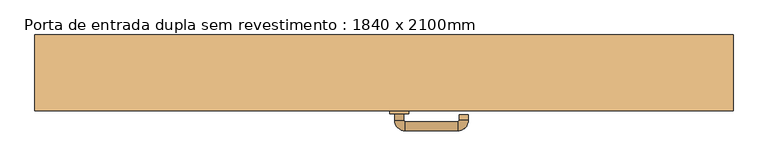
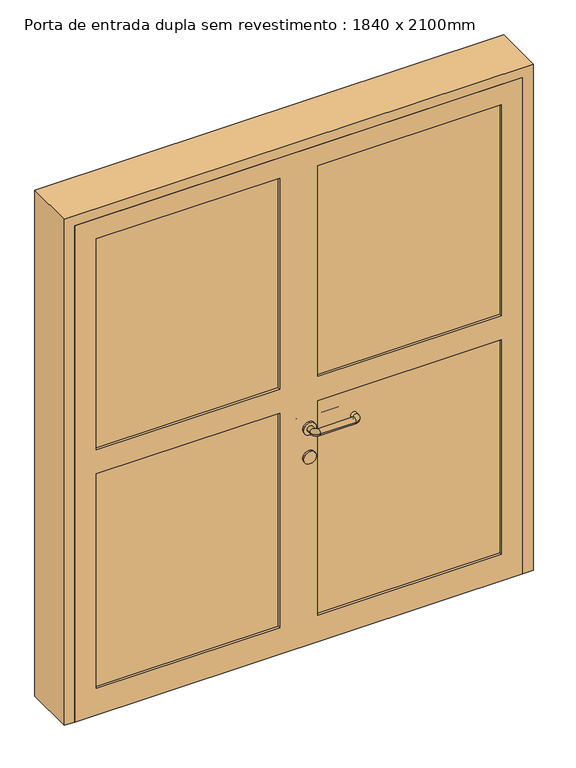
"""IFC4 building model written with IfcOpenShell, lengths in millimetres: door geometry, Porta de entrada dupla sem revestimento : 1840 x 2100mm."""

import ifcopenshell
import ifcopenshell.guid

model = None  # the IFC model being written
_history = None  # IfcOwnerHistory: only IFC2X3 demands one
_inside = {}  # id of a spatial element -> (the spatial element, [elements in it])
_under = {}  # id of a project, library or spatial element -> (it, [spatial elements below it])
_declared = {}  # id of a project -> (the project, [libraries it declares])
_typed = {}  # id of a type object -> (the type object, [elements of that type])
_made_of = {}  # id of a material, layer set ... -> (it, [elements and type objects made of it])


def new_model(schema):
    """Start an empty IFC model of exactly this schema.

    Asked for "IFC4X3", IfcOpenShell would pick the latest addendum, in which some entities
    have other attributes; the version numbers below select the first issue.
    IFC2X3 requires an IfcOwnerHistory on every rooted entity: one is made here for all.
    """
    global model, _history
    if schema == "IFC4X3":
        model = ifcopenshell.file(schema_version=(4, 3, 0, 0))
    else:
        model = ifcopenshell.file(schema=schema)
    _inside.clear()
    _under.clear()
    _declared.clear()
    _typed.clear()
    _made_of.clear()
    _history = None
    if model.schema == "IFC2X3":
        org = make("IfcOrganization", Name="unknown")
        user = make(
            "IfcPersonAndOrganization",
            ThePerson=make("IfcPerson", FamilyName="unknown"),
            TheOrganization=org,
        )
        app = make(
            "IfcApplication",
            ApplicationDeveloper=org,
            Version="unknown",
            ApplicationFullName="unknown",
            ApplicationIdentifier="unknown",
        )
        _history = make(
            "IfcOwnerHistory",
            OwningUser=user,
            OwningApplication=app,
            ChangeAction="ADDED",
            CreationDate=0,
        )
    return model


def make(cls, **values):
    """One entity of the class cls with the attributes given. An attribute that is None is left unset."""
    return model.create_entity(
        cls, **{name: value for name, value in values.items() if value is not None}
    )


def rooted(cls, **values):
    """An entity with a GlobalId (a new one), such as an element, a storey or a relation."""
    return make(cls, GlobalId=ifcopenshell.guid.new(), OwnerHistory=_history, **values)


def si_unit(unit_type, name, prefix=None):
    """IfcSIUnit, for example si_unit("LENGTHUNIT", "METRE", prefix="MILLI")."""
    return make("IfcSIUnit", UnitType=unit_type, Prefix=prefix, Name=name)


def assignment(units):
    """IfcUnitAssignment: the units of a project."""
    return None if units is None else make("IfcUnitAssignment", Units=units)


def point(xyz):
    """IfcCartesianPoint."""
    return None if xyz is None else make("IfcCartesianPoint", Coordinates=xyz)


def direction(xyz):
    """IfcDirection."""
    return None if xyz is None else make("IfcDirection", DirectionRatios=xyz)


def frame(location, z_axis=None, x_axis=None):
    """IfcAxis2Placement3D, a coordinate frame: its origin and axes. An axis left out is left unset."""
    return make(
        "IfcAxis2Placement3D",
        Location=point(location),
        Axis=direction(z_axis),
        RefDirection=direction(x_axis),
    )


def frame_2d(location, x_axis=None):
    """IfcAxis2Placement2D, a coordinate frame in the plane: its origin and x axis."""
    return make(
        "IfcAxis2Placement2D", Location=point(location), RefDirection=direction(x_axis)
    )


def origin():
    """The frame at (0, 0, 0) with its axes left unset."""
    return frame((0.0, 0.0, 0.0))


def place(relative_to, where):
    """IfcLocalPlacement: puts the frame where relative to a parent placement (None: the world)."""
    return make(
        "IfcLocalPlacement", PlacementRelTo=relative_to, RelativePlacement=where
    )


def context(
    kind, dimensions, precision=None, world=None, true_north=None, identifier=None
):
    """IfcGeometricRepresentationContext, for example the 3D "Model" context."""
    return make(
        "IfcGeometricRepresentationContext",
        ContextIdentifier=identifier,
        ContextType=kind,
        CoordinateSpaceDimension=dimensions,
        Precision=precision,
        WorldCoordinateSystem=world,
        TrueNorth=true_north,
    )


def project(units=None, contexts=None):
    """IfcProject with its units and contexts."""
    return rooted(
        "IfcProject",
        Name="project",
        RepresentationContexts=contexts,
        UnitsInContext=assignment(units),
    )


def spatial(cls, under=None, at=None, **own):
    """A site, building, storey or space (cls), placed at a placement, below another one or the project."""
    s = rooted(cls, ObjectPlacement=at, **own)
    if under is not None:
        _under.setdefault(under.id(), (under, []))[1].append(s)
    return s


def polyline(points):
    """IfcPolyline through the points."""
    return make("IfcPolyline", Points=[point(p) for p in points])


def circle_curve(where, radius):
    """IfcCircle in the frame where."""
    return make("IfcCircle", Position=where, Radius=radius)


def ellipse_curve(where, semi_axis1, semi_axis2):
    """IfcEllipse in the frame where."""
    return make(
        "IfcEllipse", Position=where, SemiAxis1=semi_axis1, SemiAxis2=semi_axis2
    )


def trimmed(basis, trim1, trim2, sense, master):
    """IfcTrimmedCurve: the piece of a basis curve between two trims."""
    return make(
        "IfcTrimmedCurve",
        BasisCurve=basis,
        Trim1=trim1,
        Trim2=trim2,
        SenseAgreement=sense,
        MasterRepresentation=master,
    )


def segment(curve, same_sense, transition):
    """IfcCompositeCurveSegment."""
    return make(
        "IfcCompositeCurveSegment",
        Transition=transition,
        SameSense=same_sense,
        ParentCurve=curve,
    )


def composite_curve(segments, self_intersect=None):
    """IfcCompositeCurve: segments joined end to end."""
    return make("IfcCompositeCurve", Segments=segments, SelfIntersect=self_intersect)


def outline(outer, holes=None, kind="AREA"):
    """IfcArbitraryClosedProfileDef: a profile drawn as a closed curve; with holes, ...WithVoids."""
    if holes is None:
        return make("IfcArbitraryClosedProfileDef", ProfileType=kind, OuterCurve=outer)
    return make(
        "IfcArbitraryProfileDefWithVoids",
        ProfileType=kind,
        OuterCurve=outer,
        InnerCurves=holes,
    )


def extrude(swept, where, along, depth):
    """IfcExtrudedAreaSolid: the profile swept, set in the frame where, extruded along a direction by depth."""
    return make(
        "IfcExtrudedAreaSolid",
        SweptArea=swept,
        Position=where,
        ExtrudedDirection=direction(along),
        Depth=depth,
    )


def faces_of(points, faces, orient=None, outer=None):
    """IfcFace entities. A face is a list of loops; a loop is a list of indices into points, from 0.

    orient and outer hold one flag for each loop. By default every Orientation is true, the
    first loop of a face is its IfcFaceOuterBound and the others are IfcFaceBound.
    """
    made = []
    for i, loops in enumerate(faces):
        bounds = []
        for j, loop in enumerate(loops):
            is_outer = j == 0 if outer is None else outer[i][j]
            bounds.append(
                make(
                    "IfcFaceOuterBound" if is_outer else "IfcFaceBound",
                    Bound=make("IfcPolyLoop", Polygon=[points[k] for k in loop]),
                    Orientation=True if orient is None else orient[i][j],
                )
            )
        made.append(make("IfcFace", Bounds=bounds))
    return made


def faceted_brep(points, faces, orient=None, outer=None, voids=None):
    """IfcFacetedBrep: a solid bounded by flat faces; with voids (closed shells), ...WithVoids."""
    shared = [point(p) for p in points]
    hull = make("IfcClosedShell", CfsFaces=faces_of(shared, faces, orient, outer))
    if voids is None:
        return make("IfcFacetedBrep", Outer=hull)
    return make(
        "IfcFacetedBrepWithVoids",
        Outer=hull,
        Voids=[
            make(cls, CfsFaces=faces_of(shared, fs, o, b)) for cls, fs, o, b in voids
        ],
    )


def shape(context_of_items, identifier, shape_type, items):
    """IfcShapeRepresentation: the items that make up one representation, for example the "Body"."""
    return make(
        "IfcShapeRepresentation",
        ContextOfItems=context_of_items,
        RepresentationIdentifier=identifier,
        RepresentationType=shape_type,
        Items=items,
    )


def source(mapping_origin, context_of_items, identifier, shape_type, items):
    """IfcRepresentationMap: a shape defined once, which mapped items show again and again."""
    return make(
        "IfcRepresentationMap",
        MappingOrigin=mapping_origin,
        MappedRepresentation=shape(context_of_items, identifier, shape_type, items),
    )


def transform(
    local_origin,
    x_axis=None,
    y_axis=None,
    z_axis=None,
    scale=None,
    scale2=None,
    scale3=None,
    uniform=True,
):
    """IfcCartesianTransformationOperator3D, or its non-uniform kind. x_axis, y_axis, z_axis: its Axis1, 2, 3."""
    if uniform:
        return make(
            "IfcCartesianTransformationOperator3D",
            Axis1=direction(x_axis),
            Axis2=direction(y_axis),
            LocalOrigin=point(local_origin),
            Scale=scale,
            Axis3=direction(z_axis),
        )
    return make(
        "IfcCartesianTransformationOperator3DnonUniform",
        Axis1=direction(x_axis),
        Axis2=direction(y_axis),
        LocalOrigin=point(local_origin),
        Scale=scale,
        Axis3=direction(z_axis),
        Scale2=scale2,
        Scale3=scale3,
    )


def mapped(mapping_source, mapping_target):
    """IfcMappedItem: shows the shape of a source again, moved by a transform."""
    return make(
        "IfcMappedItem", MappingSource=mapping_source, MappingTarget=mapping_target
    )


def made_of(thing, what):
    """Note that an element or type object is made of a material, layer set ...; save() writes the relation."""
    if what is not None:
        _made_of.setdefault(what.id(), (what, []))[1].append(thing)
    return thing


def element(
    cls,
    number,
    at=None,
    inside=None,
    cuts=None,
    type_object=None,
    material=None,
    context=None,
    identifier="Body",
    shape_type=None,
    held_by="IfcProductDefinitionShape",
    body=None,
    shapes=None,
    **own,
):
    """One element of the class cls, such as IfcWall. Its Tag is "e" and its number.

    at: its placement. inside: the storey or other place that contains it. cuts: it is an
    opening in that element (IfcRelVoidsElement). A single representation is given by context,
    identifier, shape_type and body (its items); several are given by shapes. held_by: the class
    of the entity that holds the representations. save() writes the other relations.
    """
    e = rooted(cls, Tag="e%d" % number, ObjectPlacement=at, **own)
    if body is not None:
        shapes = [shape(context, identifier, shape_type, body)]
    if shapes is not None:
        e.Representation = make(held_by, Representations=shapes)
    if inside is not None:
        _inside.setdefault(inside.id(), (inside, []))[1].append(e)
    if cuts is not None:
        rooted(
            "IfcRelVoidsElement", RelatingBuildingElement=cuts, RelatedOpeningElement=e
        )
    if type_object is not None:
        _typed.setdefault(type_object.id(), (type_object, []))[1].append(e)
    return made_of(e, material)


def aggregate(whole, parts):
    """IfcRelAggregates: a whole, such as a stair, and the parts it consists of."""
    return rooted("IfcRelAggregates", RelatingObject=whole, RelatedObjects=parts)


def save(model, path):
    """Write the relations noted so far, then the file.

    IfcRelAggregates (storeys below a building ...), IfcRelContainedInSpatialStructure (elements
    in a storey), IfcRelDefinesByType, IfcRelAssociatesMaterial and IfcRelDeclares: one each for
    every whole, place, type object, material and project.
    """
    for whole, parts in _under.values():
        aggregate(whole, parts)
    for where, things in _inside.values():
        rooted(
            "IfcRelContainedInSpatialStructure",
            RelatedElements=things,
            RelatingStructure=where,
        )
    for kind, things in _typed.values():
        rooted("IfcRelDefinesByType", RelatedObjects=things, RelatingType=kind)
    for what, things in _made_of.values():
        rooted("IfcRelAssociatesMaterial", RelatedObjects=things, RelatingMaterial=what)
    for by, libraries in _declared.values():
        rooted("IfcRelDeclares", RelatingContext=by, RelatedDefinitions=libraries)
    model.write(path)


def plane_surface(at):
    """IfcPlane: the flat surface through the origin of the frame at, square to its z axis."""
    return make("IfcPlane", Position=at)


def cylinder_surface(at, radius):
    """IfcCylindricalSurface: all points at the distance radius from the z axis of the frame at."""
    return make("IfcCylindricalSurface", Position=at, Radius=radius)


def revolved_surface(curve, axis_point, axis_direction):
    """IfcSurfaceOfRevolution: the curve turned about the line through axis_point along axis_direction."""
    return make(
        "IfcSurfaceOfRevolution",
        SweptCurve=make("IfcArbitraryOpenProfileDef", ProfileType="CURVE", Curve=curve),
        AxisPosition=make("IfcAxis1Placement", Location=point(axis_point), Axis=direction(axis_direction)),
    )


def advanced_brep(points, edges, surfaces, faces):
    """IfcAdvancedBrep: a solid bounded by faces that lie on surfaces and meet in shared edges.

    An edge is (start, end): straight between two places in points (the first is 0);
    or (start, end, curve); or (start, end, curve, False) where it runs against its curve.
    A face is (place in surfaces, loops), or (place, loops, False) where it looks against
    its surface's normal. A loop lists edges by number (the first is 1), with a minus sign
    where the edge is run from its end to its start. The first loop is the outer one.
    """
    corners = [point(p) for p in points]
    vertices = [make("IfcVertexPoint", VertexGeometry=c) for c in corners]
    made = []
    for start, end, *more in edges:
        made.append(
            make(
                "IfcEdgeCurve",
                EdgeStart=vertices[start],
                EdgeEnd=vertices[end],
                EdgeGeometry=more[0] if more else make("IfcPolyline", Points=[corners[start], corners[end]]),
                SameSense=more[1] if len(more) > 1 else True,
            )
        )
    hull = []
    for where, loops, *sense in faces:
        bounds = []
        for j, loop in enumerate(loops):
            ring = [make("IfcOrientedEdge", EdgeElement=made[abs(k) - 1], Orientation=k > 0) for k in loop]
            bounds.append(
                make(
                    "IfcFaceOuterBound" if j == 0 else "IfcFaceBound",
                    Bound=make("IfcEdgeLoop", EdgeList=ring),
                    Orientation=True,
                )
            )
        hull.append(make("IfcAdvancedFace", Bounds=bounds, FaceSurface=surfaces[where], SameSense=sense[0] if sense else True))
    return make("IfcAdvancedBrep", Outer=make("IfcClosedShell", CfsFaces=hull))


def porta_de_entrada_dupla_sem_revestimento_1840_x_2100mm_60e580c7(model_context):
    return source(origin(), model_context, "Body", "SolidModel", [
        advanced_brep(
        [(52.0, -57.0, 900.0), (28.0, -57.0, 900.0), (52.0, -40.0, 900.0), (28.0, -40.0, 900.0), (55.0, -13.0, 900.0), (55.0, -37.0, 900.0), (195.0, -37.0, 900.0), (195.0, -13.0, 900.0), (222.0, -40.0, 900.0), (198.0, -40.0, 900.0), (198.0, -55.0, 900.0), (222.0, -55.0, 900.0)],
        [
            (0, 1, circle_curve(frame((40.0, -57.0, 900.0), z_axis=(0.0, -1.0, 0.0), x_axis=(-1.0, 0.0, 0.0)), 12.0)),
            (1, 0, circle_curve(frame((40.0, -57.0, 900.0), z_axis=(0.0, -1.0, 0.0), x_axis=(-1.0, 0.0, 0.0)), 12.0)),
            (0, 2),
            (2, 3, circle_curve(frame((40.0, -40.0, 900.0), z_axis=(0.0, -1.0, 0.0), x_axis=(-1.0, 0.0, 0.0)), 12.0)),
            (3, 1),
            (3, 2, circle_curve(frame((40.0, -40.0, 900.0), z_axis=(0.0, -1.0, 0.0), x_axis=(-1.0, 0.0, 0.0)), 12.0)),
            (4, 3, circle_curve(frame((55.0, -40.0, 900.0), z_axis=(0.0, 0.0, 1.0), x_axis=(-1.0, 0.0, 0.0)), 27.0)),
            (2, 5, circle_curve(frame((55.0, -40.0, 900.0), z_axis=(0.0, 0.0, -1.0), x_axis=(-1.0, 0.0, 0.0)), 3.0)),
            (5, 4, circle_curve(frame((55.0, -25.0, 900.0), z_axis=(-1.0, 0.0, 0.0), x_axis=(0.0, 1.0, 0.0)), 12.0)),
            (4, 5, circle_curve(frame((55.0, -25.0, 900.0), z_axis=(-1.0, 0.0, 0.0), x_axis=(0.0, 1.0, 0.0)), 12.0)),
            (5, 6),
            (6, 7, circle_curve(frame((195.0, -25.0, 900.0), z_axis=(-1.0, 0.0, 0.0), x_axis=(0.0, 1.0, 0.0)), 12.0)),
            (7, 4),
            (7, 6, circle_curve(frame((195.0, -25.0, 900.0), z_axis=(-1.0, 0.0, 0.0), x_axis=(0.0, 1.0, 0.0)), 12.0)),
            (8, 7, circle_curve(frame((195.0, -40.0, 900.0), z_axis=(0.0, 0.0, 1.0), x_axis=(0.0, 1.0, 0.0)), 27.0)),
            (6, 9, circle_curve(frame((195.0, -40.0, 900.0), z_axis=(0.0, 0.0, -1.0), x_axis=(0.0, 1.0, 0.0)), 3.0)),
            (9, 8, circle_curve(frame((210.0, -40.0, 900.0), z_axis=(0.0, 1.0, 0.0), x_axis=(1.0, 0.0, 0.0)), 12.0)),
            (8, 9, circle_curve(frame((210.0, -40.0, 900.0), z_axis=(0.0, 1.0, 0.0), x_axis=(1.0, 0.0, 0.0)), 12.0)),
            (10, 11, circle_curve(frame((210.0, -55.0, 900.0), z_axis=(0.0, -1.0, 0.0), x_axis=(1.0, 0.0, 0.0)), 12.0)),
            (11, 10, circle_curve(frame((210.0, -55.0, 900.0), z_axis=(0.0, -1.0, 0.0), x_axis=(1.0, 0.0, 0.0)), 12.0)),
            (9, 10),
            (11, 8),
        ],
        [
            plane_surface(frame((-802.0, -57.0, 1730.0), z_axis=(0.0, -1.0, 0.0), x_axis=(0.0, 0.0, 1.0))),
            cylinder_surface(frame((40.0, -57.0, 900.0), z_axis=(0.0, -1.0, 0.0), x_axis=(-1.0, 0.0, 0.0)), 12.0),
            revolved_surface(trimmed(ellipse_curve(frame((40.0, -40.0, 900.0), z_axis=(0.0, -1.0, 0.0), x_axis=(-1.0, 0.0, 0.0)), 12.0, 12.0), [point((52.0, -40.0, 900.0))], [point((28.0, -40.0, 900.0))], True, "CARTESIAN"), (55.0, -40.0, 1730.0), (0.0, 0.0, -1.0)),
            revolved_surface(trimmed(ellipse_curve(frame((40.0, -40.0, 900.0), z_axis=(0.0, -1.0, 0.0), x_axis=(-1.0, 0.0, 0.0)), 12.0, 12.0), [point((28.0, -40.0, 900.0))], [point((52.0, -40.0, 900.0))], True, "CARTESIAN"), (55.0, -40.0, 1730.0), (0.0, 0.0, -1.0)),
            cylinder_surface(frame((55.0, -25.0, 900.0), z_axis=(-1.0, 0.0, 0.0), x_axis=(0.0, 1.0, 0.0)), 12.0),
            revolved_surface(trimmed(ellipse_curve(frame((195.0, -25.0, 900.0), z_axis=(-1.0, 0.0, 0.0), x_axis=(0.0, 1.0, 0.0)), 12.0, 12.0), [point((195.0, -37.0, 900.0))], [point((195.0, -13.0, 900.0))], True, "CARTESIAN"), (195.0, -40.0, 1730.0), (0.0, 0.0, -1.0)),
            revolved_surface(trimmed(ellipse_curve(frame((195.0, -25.0, 900.0), z_axis=(-1.0, 0.0, 0.0), x_axis=(0.0, 1.0, 0.0)), 12.0, 12.0), [point((195.0, -13.0, 900.0))], [point((195.0, -37.0, 900.0))], True, "CARTESIAN"), (195.0, -40.0, 1730.0), (0.0, 0.0, -1.0)),
            plane_surface(frame((-632.0, -55.0, 1730.0), z_axis=(0.0, -1.0, 0.0), x_axis=(0.0, 0.0, -1.0))),
            cylinder_surface(frame((210.0, -40.0, 900.0), z_axis=(0.0, 1.0, 0.0), x_axis=(1.0, 0.0, 0.0)), 12.0),
        ],
        [
            (0, [[1, 2]]),
            (1, [[-1, 3, 4, 5]]),
            (1, [[-2, -5, 6, -3]]),
            (2, [[7, -4, 8, 9]]),
            (3, [[-8, -6, -7, 10]]),
            (4, [[-9, 11, 12, 13]]),
            (4, [[-10, -13, 14, -11]]),
            (5, [[15, -12, 16, 17]]),
            (6, [[-16, -14, -15, 18]]),
            (7, [[19, 20]]),
            (8, [[-17, 21, -20, 22]]),
            (8, [[-18, -22, -19, -21]]),
        ],
    ),
        extrude(outline(composite_curve([segment(trimmed(circle_curve(frame_2d((780.0, 40.0)), 25.0), [point((780.0, 15.0))], [point((780.0, 65.0))], False, "CARTESIAN"), True, "CONTINUOUS"), segment(trimmed(circle_curve(frame_2d((780.0, 40.0)), 25.0), [point((780.0, 65.0))], [point((780.0, 15.0))], False, "CARTESIAN"), True, "CONTINUOUS")], self_intersect=False)), frame((0.0, -65.0, 0.0), z_axis=(0.0, 1.0, 0.0), x_axis=(0.0, 0.0, 1.0)), (0.0, 0.0, 1.0), 8.0),
        extrude(outline(composite_curve([segment(trimmed(circle_curve(frame_2d((900.0, 40.0)), 25.0), [point((900.0, 15.0))], [point((900.0, 65.0))], False, "CARTESIAN"), True, "CONTINUOUS"), segment(trimmed(circle_curve(frame_2d((900.0, 40.0)), 25.0), [point((900.0, 65.0))], [point((900.0, 15.0))], False, "CARTESIAN"), True, "CONTINUOUS")], self_intersect=False)), frame((0.0, -65.0, 0.0), z_axis=(0.0, 1.0, 0.0), x_axis=(0.0, 0.0, 1.0)), (0.0, 0.0, 1.0), 8.0),
        advanced_brep(
        [(28.0, -108.0, 900.0), (52.0, -108.0, 900.0), (28.0, -125.0, 900.0), (52.0, -125.0, 900.0), (55.0, -128.0, 900.0), (55.0, -152.0, 900.0), (195.0, -152.0, 900.0), (195.0, -128.0, 900.0), (198.0, -125.0, 900.0), (222.0, -125.0, 900.0), (222.0, -110.0, 900.0), (198.0, -110.0, 900.0)],
        [
            (0, 1, circle_curve(frame((40.0, -108.0, 900.0), z_axis=(0.0, 1.0, 0.0), x_axis=(1.0, 0.0, 0.0)), 12.0)),
            (1, 0, circle_curve(frame((40.0, -108.0, 900.0), z_axis=(0.0, 1.0, 0.0), x_axis=(1.0, 0.0, 0.0)), 12.0)),
            (0, 2),
            (2, 3, circle_curve(frame((40.0, -125.0, 900.0), z_axis=(0.0, 1.0, 0.0), x_axis=(1.0, 0.0, 0.0)), 12.0)),
            (3, 1),
            (3, 2, circle_curve(frame((40.0, -125.0, 900.0), z_axis=(0.0, 1.0, 0.0), x_axis=(1.0, 0.0, 0.0)), 12.0)),
            (4, 3, circle_curve(frame((55.0, -125.0, 900.0), z_axis=(0.0, 0.0, -1.0), x_axis=(-1.0, 0.0, 0.0)), 3.0)),
            (2, 5, circle_curve(frame((55.0, -125.0, 900.0), z_axis=(0.0, 0.0, 1.0), x_axis=(-1.0, 0.0, 0.0)), 27.0)),
            (5, 4, circle_curve(frame((55.0, -140.0, 900.0), z_axis=(-1.0, 0.0, 0.0), x_axis=(0.0, 1.0, 0.0)), 12.0)),
            (4, 5, circle_curve(frame((55.0, -140.0, 900.0), z_axis=(-1.0, 0.0, 0.0), x_axis=(0.0, 1.0, 0.0)), 12.0)),
            (5, 6),
            (6, 7, circle_curve(frame((195.0, -140.0, 900.0), z_axis=(-1.0, 0.0, 0.0), x_axis=(0.0, 1.0, 0.0)), 12.0)),
            (7, 4),
            (7, 6, circle_curve(frame((195.0, -140.0, 900.0), z_axis=(-1.0, 0.0, 0.0), x_axis=(0.0, 1.0, 0.0)), 12.0)),
            (8, 7, circle_curve(frame((195.0, -125.0, 900.0), z_axis=(0.0, 0.0, -1.0), x_axis=(0.0, -1.0, 0.0)), 3.0)),
            (6, 9, circle_curve(frame((195.0, -125.0, 900.0), z_axis=(0.0, 0.0, 1.0), x_axis=(0.0, -1.0, 0.0)), 27.0)),
            (9, 8, circle_curve(frame((210.0, -125.0, 900.0), z_axis=(0.0, -1.0, 0.0), x_axis=(-1.0, 0.0, 0.0)), 12.0)),
            (8, 9, circle_curve(frame((210.0, -125.0, 900.0), z_axis=(0.0, -1.0, 0.0), x_axis=(-1.0, 0.0, 0.0)), 12.0)),
            (10, 11, circle_curve(frame((210.0, -110.0, 900.0), z_axis=(0.0, 1.0, 0.0), x_axis=(-1.0, 0.0, 0.0)), 12.0)),
            (11, 10, circle_curve(frame((210.0, -110.0, 900.0), z_axis=(0.0, 1.0, 0.0), x_axis=(-1.0, 0.0, 0.0)), 12.0)),
            (9, 10),
            (11, 8),
        ],
        [
            plane_surface(frame((-802.0, -108.0, 1730.0), z_axis=(0.0, 1.0, 0.0), x_axis=(0.0, 0.0, -1.0))),
            cylinder_surface(frame((40.0, -108.0, 900.0), z_axis=(0.0, 1.0, 0.0), x_axis=(1.0, 0.0, 0.0)), 12.0),
            revolved_surface(trimmed(ellipse_curve(frame((40.0, -125.0, 900.0), z_axis=(0.0, 1.0, 0.0), x_axis=(1.0, 0.0, 0.0)), 12.0, 12.0), [point((28.0, -125.0, 900.0))], [point((52.0, -125.0, 900.0))], True, "CARTESIAN"), (55.0, -125.0, 1730.0), (0.0, 0.0, 1.0)),
            revolved_surface(trimmed(ellipse_curve(frame((40.0, -125.0, 900.0), z_axis=(0.0, 1.0, 0.0), x_axis=(1.0, 0.0, 0.0)), 12.0, 12.0), [point((52.0, -125.0, 900.0))], [point((28.0, -125.0, 900.0))], True, "CARTESIAN"), (55.0, -125.0, 1730.0), (0.0, 0.0, 1.0)),
            cylinder_surface(frame((55.0, -140.0, 900.0), z_axis=(-1.0, 0.0, 0.0), x_axis=(0.0, 1.0, 0.0)), 12.0),
            revolved_surface(trimmed(ellipse_curve(frame((195.0, -140.0, 900.0), z_axis=(-1.0, 0.0, 0.0), x_axis=(0.0, 1.0, 0.0)), 12.0, 12.0), [point((195.0, -152.0, 900.0))], [point((195.0, -128.0, 900.0))], True, "CARTESIAN"), (195.0, -125.0, 1730.0), (0.0, 0.0, 1.0)),
            revolved_surface(trimmed(ellipse_curve(frame((195.0, -140.0, 900.0), z_axis=(-1.0, 0.0, 0.0), x_axis=(0.0, 1.0, 0.0)), 12.0, 12.0), [point((195.0, -128.0, 900.0))], [point((195.0, -152.0, 900.0))], True, "CARTESIAN"), (195.0, -125.0, 1730.0), (0.0, 0.0, 1.0)),
            plane_surface(frame((-632.0, -110.0, 1730.0), z_axis=(0.0, 1.0, 0.0), x_axis=(0.0, 0.0, 1.0))),
            cylinder_surface(frame((210.0, -125.0, 900.0), z_axis=(0.0, -1.0, 0.0), x_axis=(-1.0, 0.0, 0.0)), 12.0),
        ],
        [
            (0, [[1, 2]]),
            (1, [[-1, 3, 4, 5]]),
            (1, [[-2, -5, 6, -3]]),
            (2, [[7, -4, 8, 9]]),
            (3, [[-8, -6, -7, 10]]),
            (4, [[-9, 11, 12, 13]]),
            (4, [[-10, -13, 14, -11]]),
            (5, [[15, -12, 16, 17]]),
            (6, [[-16, -14, -15, 18]]),
            (7, [[19, 20]]),
            (8, [[-17, 21, -20, 22]]),
            (8, [[-18, -22, -19, -21]]),
        ],
    ),
        extrude(outline(composite_curve([segment(trimmed(circle_curve(frame_2d((780.0, 40.0)), 25.0), [point((780.0, 15.0))], [point((780.0, 65.0))], False, "CARTESIAN"), True, "CONTINUOUS"), segment(trimmed(circle_curve(frame_2d((780.0, 40.0)), 25.0), [point((780.0, 65.0))], [point((780.0, 15.0))], False, "CARTESIAN"), True, "CONTINUOUS")], self_intersect=False)), frame((0.0, -108.0, 0.0), z_axis=(0.0, 1.0, 0.0), x_axis=(0.0, 0.0, 1.0)), (0.0, 0.0, 1.0), 8.0),
        extrude(outline(composite_curve([segment(trimmed(circle_curve(frame_2d((900.0, 40.0)), 25.0), [point((900.0, 15.0))], [point((900.0, 65.0))], False, "CARTESIAN"), True, "CONTINUOUS"), segment(trimmed(circle_curve(frame_2d((900.0, 40.0)), 25.0), [point((900.0, 65.0))], [point((900.0, 15.0))], False, "CARTESIAN"), True, "CONTINUOUS")], self_intersect=False)), frame((0.0, -108.0, 0.0), z_axis=(0.0, 1.0, 0.0), x_axis=(0.0, 0.0, 1.0)), (0.0, 0.0, 1.0), 8.0),
        extrude(outline(polyline([(-835.0, -75.5), (835.0, -75.5), (835.0, -89.5), (-835.0, -89.5), (-835.0, -75.5)])), frame((0.0, 0.0, 70.0), z_axis=(0.0, 0.0, 1.0), x_axis=(1.0, 0.0, 0.0)), (0.0, 0.0, 1.0), 970.0),
        extrude(outline(polyline([(-835.0, -75.5), (835.0, -75.5), (835.0, -89.5), (-835.0, -89.5), (-835.0, -75.5)])), frame((0.0, 0.0, 1060.0), z_axis=(0.0, 0.0, 1.0), x_axis=(1.0, 0.0, 0.0)), (0.0, 0.0, 1.0), 955.0),
        extrude(outline(polyline([(-835.0, -75.5), (835.0, -75.5), (835.0, -89.5), (-835.0, -89.5), (-835.0, -75.5)])), frame((0.0, 0.0, 70.0), z_axis=(0.0, 0.0, 1.0), x_axis=(1.0, 0.0, 0.0)), (0.0, 0.0, 1.0), 970.0),
        extrude(outline(polyline([(-835.0, -75.5), (835.0, -75.5), (835.0, -89.5), (-835.0, -89.5), (-835.0, -75.5)])), frame((0.0, 0.0, 1060.0), z_axis=(0.0, 0.0, 1.0), x_axis=(1.0, 0.0, 0.0)), (0.0, 0.0, 1.0), 955.0),
        faceted_brep([(-920.0, 100.0, 0.0), (-870.0, 100.0, 0.0), (-870.0, -62.0, 0.0), (-880.0, -62.0, 0.0), (-880.0, -100.0, 0.0), (-920.0, -100.0, 0.0), (-920.0, 100.0, 2100.0), (920.0, 100.0, 2100.0), (920.0, 100.0, 0.0), (870.0, 100.0, 0.0), (870.0, 100.0, 2050.0), (-870.0, 100.0, 2050.0), (-870.0, -62.0, 2050.0), (870.0, -62.0, 2050.0), (870.0, -62.0, 0.0), (880.0, -62.0, 0.0), (880.0, -62.0, 2060.0), (-880.0, -62.0, 2060.0), (-880.0, -100.0, 2060.0), (880.0, -100.0, 2060.0), (880.0, -100.0, 0.0), (920.0, -100.0, 0.0), (920.0, -100.0, 2100.0), (-920.0, -100.0, 2100.0)], [[[0, 1, 2, 3, 4, 5]], [[1, 0, 6, 7, 8, 9, 10, 11]], [[2, 1, 11, 12]], [[3, 2, 12, 13, 14, 15, 16, 17]], [[4, 3, 17, 18]], [[5, 4, 18, 19, 20, 21, 22, 23]], [[0, 5, 23, 6]], [[7, 22, 21, 8]], [[8, 21, 20, 15, 14, 9]], [[13, 10, 9, 14]], [[19, 16, 15, 20]], [[12, 11, 10, 13]], [[18, 17, 16, 19]], [[6, 23, 22, 7]]]),
        extrude(outline(polyline([(2060.0, -880.0), (0.0, -880.0), (0.0, 880.0), (2060.0, 880.0), (2060.0, -880.0)]), holes=[polyline([(1975.0, 75.0), (1975.0, 795.0), (1100.0, 795.0), (1100.0, 75.0), (1975.0, 75.0)]), polyline([(1100.0, -795.0), (1975.0, -795.0), (1975.0, -75.0), (1100.0, -75.0), (1100.0, -795.0)]), polyline([(1000.0, 795.0), (110.0, 795.0), (110.0, 75.0), (1000.0, 75.0), (1000.0, 795.0)]), polyline([(110.0, -75.0), (110.0, -795.0), (1000.0, -795.0), (1000.0, -75.0), (110.0, -75.0)])]), frame((0.0, -100.0, 0.0), z_axis=(0.0, 1.0, 0.0), x_axis=(0.0, 0.0, 1.0)), (0.0, 0.0, 1.0), 35.0),
    ])


if __name__ == "__main__":
    model = new_model("IFC4")
    model_context = context("Model", 3, world=origin())
    ifc_project = project(units=[si_unit("LENGTHUNIT", "METRE", prefix="MILLI")], contexts=[model_context])
    site = spatial("IfcSite", under=ifc_project)
    building = spatial("IfcBuilding", under=site)
    placement = place(None, origin())
    porta_de_entrada_dupla_sem_revestimento_1840_x_2100mm_shape = porta_de_entrada_dupla_sem_revestimento_1840_x_2100mm_60e580c7(model_context)
    element("IfcDoor", 1, ObjectType="Porta de entrada dupla sem revestimento : 1840 x 2100mm", at=placement, inside=building, context=model_context, shape_type="MappedRepresentation", body=[
        mapped(porta_de_entrada_dupla_sem_revestimento_1840_x_2100mm_shape, transform((0.0, 0.0, 0.0), x_axis=(1.0, 0.0, 0.0), y_axis=(0.0, 1.0, 0.0), z_axis=(0.0, 0.0, 1.0))),
    ])
    save(model, "model.ifc")

# Revit data of these elements
# Type "Porta de entrada dupla sem revestimento : 1840 x 2100mm"
#   Type Mark = "40"
#   Construction Type Id = "MDOOR"
#   Analytic Construction = "Metal"
#   W2 = 0.920 m
#   W1 = 1.760 m
#   Thickness = 0.035 m
#   Rough Width = 1.840 m
#   Rough Height = 2.100 m
#   Largura da moldura do painel = 0.075 m
#   Heat Transfer Coefficient (U) = 3.7021 W/(m²·K)
#   Largura da estrutura = 0.050 m
#   Height = 2.100 m
#   Width = 1.840 m
#   Define Thermal Properties by = 1
#   Function = 1
#   Material do painel = none
#   Material do puxador = none
#   Vidro = none
#   Material da moldura = none
#   Visual Light Transmittance = 0
#   Solar Heat Gain Coefficient = 0
#   Wall Closure = (empty or 0)
# Element 1 (IfcDoor, "Porta de entrada dupla sem revestimento : 1840 x 2100mm")
#   Materials on its faces: "Vidro"
# Materials
#   "Vidro": class "Vidro", colour RGB 0 128 192, transparency 0.9, Description = "Vidro de sílica", Cost = 0
